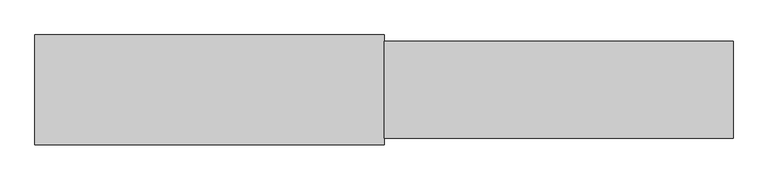
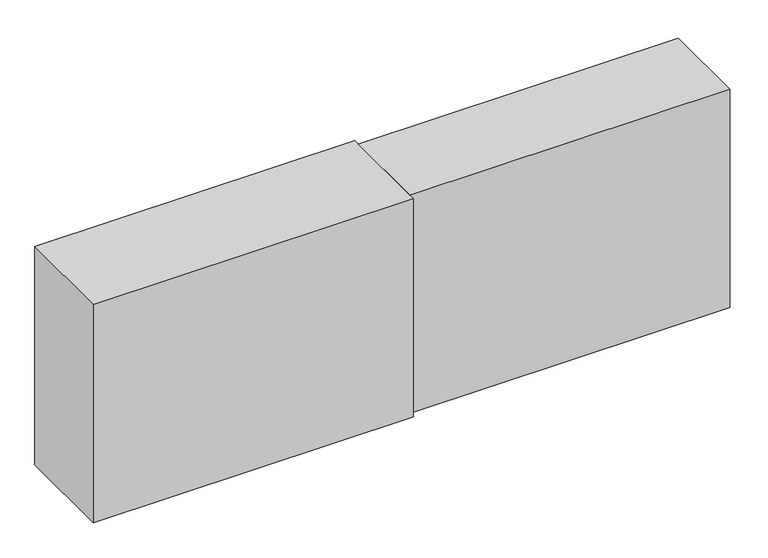
"""IFC4 building model written with IfcOpenShell, lengths in millimetres: proxy geometry, Тепловой пункт : Тепловой пункт."""

import ifcopenshell
import ifcopenshell.guid

model = None  # the IFC model being written
_history = None  # IfcOwnerHistory: only IFC2X3 demands one
_inside = {}  # id of a spatial element -> (the spatial element, [elements in it])
_under = {}  # id of a project, library or spatial element -> (it, [spatial elements below it])
_declared = {}  # id of a project -> (the project, [libraries it declares])
_typed = {}  # id of a type object -> (the type object, [elements of that type])
_made_of = {}  # id of a material, layer set ... -> (it, [elements and type objects made of it])


def new_model(schema):
    """Start an empty IFC model of exactly this schema.

    Asked for "IFC4X3", IfcOpenShell would pick the latest addendum, in which some entities
    have other attributes; the version numbers below select the first issue.
    IFC2X3 requires an IfcOwnerHistory on every rooted entity: one is made here for all.
    """
    global model, _history
    if schema == "IFC4X3":
        model = ifcopenshell.file(schema_version=(4, 3, 0, 0))
    else:
        model = ifcopenshell.file(schema=schema)
    _inside.clear()
    _under.clear()
    _declared.clear()
    _typed.clear()
    _made_of.clear()
    _history = None
    if model.schema == "IFC2X3":
        org = make("IfcOrganization", Name="unknown")
        user = make(
            "IfcPersonAndOrganization",
            ThePerson=make("IfcPerson", FamilyName="unknown"),
            TheOrganization=org,
        )
        app = make(
            "IfcApplication",
            ApplicationDeveloper=org,
            Version="unknown",
            ApplicationFullName="unknown",
            ApplicationIdentifier="unknown",
        )
        _history = make(
            "IfcOwnerHistory",
            OwningUser=user,
            OwningApplication=app,
            ChangeAction="ADDED",
            CreationDate=0,
        )
    return model


def make(cls, **values):
    """One entity of the class cls with the attributes given. An attribute that is None is left unset."""
    return model.create_entity(
        cls, **{name: value for name, value in values.items() if value is not None}
    )


def rooted(cls, **values):
    """An entity with a GlobalId (a new one), such as an element, a storey or a relation."""
    return make(cls, GlobalId=ifcopenshell.guid.new(), OwnerHistory=_history, **values)


def si_unit(unit_type, name, prefix=None):
    """IfcSIUnit, for example si_unit("LENGTHUNIT", "METRE", prefix="MILLI")."""
    return make("IfcSIUnit", UnitType=unit_type, Prefix=prefix, Name=name)


def assignment(units):
    """IfcUnitAssignment: the units of a project."""
    return None if units is None else make("IfcUnitAssignment", Units=units)


def point(xyz):
    """IfcCartesianPoint."""
    return None if xyz is None else make("IfcCartesianPoint", Coordinates=xyz)


def direction(xyz):
    """IfcDirection."""
    return None if xyz is None else make("IfcDirection", DirectionRatios=xyz)


def frame(location, z_axis=None, x_axis=None):
    """IfcAxis2Placement3D, a coordinate frame: its origin and axes. An axis left out is left unset."""
    return make(
        "IfcAxis2Placement3D",
        Location=point(location),
        Axis=direction(z_axis),
        RefDirection=direction(x_axis),
    )


def origin():
    """The frame at (0, 0, 0) with its axes left unset."""
    return frame((0.0, 0.0, 0.0))


def origin_with_axes():
    """The frame at (0, 0, 0) with the z axis (0, 0, 1) and the x axis (1, 0, 0) written out."""
    return frame((0.0, 0.0, 0.0), z_axis=(0.0, 0.0, 1.0), x_axis=(1.0, 0.0, 0.0))


def place(relative_to, where):
    """IfcLocalPlacement: puts the frame where relative to a parent placement (None: the world)."""
    return make(
        "IfcLocalPlacement", PlacementRelTo=relative_to, RelativePlacement=where
    )


def context(
    kind, dimensions, precision=None, world=None, true_north=None, identifier=None
):
    """IfcGeometricRepresentationContext, for example the 3D "Model" context."""
    return make(
        "IfcGeometricRepresentationContext",
        ContextIdentifier=identifier,
        ContextType=kind,
        CoordinateSpaceDimension=dimensions,
        Precision=precision,
        WorldCoordinateSystem=world,
        TrueNorth=true_north,
    )


def project(units=None, contexts=None):
    """IfcProject with its units and contexts."""
    return rooted(
        "IfcProject",
        Name="project",
        RepresentationContexts=contexts,
        UnitsInContext=assignment(units),
    )


def spatial(cls, under=None, at=None, **own):
    """A site, building, storey or space (cls), placed at a placement, below another one or the project."""
    s = rooted(cls, ObjectPlacement=at, **own)
    if under is not None:
        _under.setdefault(under.id(), (under, []))[1].append(s)
    return s


def polyline(points):
    """IfcPolyline through the points."""
    return make("IfcPolyline", Points=[point(p) for p in points])


def outline(outer, holes=None, kind="AREA"):
    """IfcArbitraryClosedProfileDef: a profile drawn as a closed curve; with holes, ...WithVoids."""
    if holes is None:
        return make("IfcArbitraryClosedProfileDef", ProfileType=kind, OuterCurve=outer)
    return make(
        "IfcArbitraryProfileDefWithVoids",
        ProfileType=kind,
        OuterCurve=outer,
        InnerCurves=holes,
    )


def extrude(swept, where, along, depth):
    """IfcExtrudedAreaSolid: the profile swept, set in the frame where, extruded along a direction by depth."""
    return make(
        "IfcExtrudedAreaSolid",
        SweptArea=swept,
        Position=where,
        ExtrudedDirection=direction(along),
        Depth=depth,
    )


def shape(context_of_items, identifier, shape_type, items):
    """IfcShapeRepresentation: the items that make up one representation, for example the "Body"."""
    return make(
        "IfcShapeRepresentation",
        ContextOfItems=context_of_items,
        RepresentationIdentifier=identifier,
        RepresentationType=shape_type,
        Items=items,
    )


def source(mapping_origin, context_of_items, identifier, shape_type, items):
    """IfcRepresentationMap: a shape defined once, which mapped items show again and again."""
    return make(
        "IfcRepresentationMap",
        MappingOrigin=mapping_origin,
        MappedRepresentation=shape(context_of_items, identifier, shape_type, items),
    )


def transform(
    local_origin,
    x_axis=None,
    y_axis=None,
    z_axis=None,
    scale=None,
    scale2=None,
    scale3=None,
    uniform=True,
):
    """IfcCartesianTransformationOperator3D, or its non-uniform kind. x_axis, y_axis, z_axis: its Axis1, 2, 3."""
    if uniform:
        return make(
            "IfcCartesianTransformationOperator3D",
            Axis1=direction(x_axis),
            Axis2=direction(y_axis),
            LocalOrigin=point(local_origin),
            Scale=scale,
            Axis3=direction(z_axis),
        )
    return make(
        "IfcCartesianTransformationOperator3DnonUniform",
        Axis1=direction(x_axis),
        Axis2=direction(y_axis),
        LocalOrigin=point(local_origin),
        Scale=scale,
        Axis3=direction(z_axis),
        Scale2=scale2,
        Scale3=scale3,
    )


def mapped(mapping_source, mapping_target):
    """IfcMappedItem: shows the shape of a source again, moved by a transform."""
    return make(
        "IfcMappedItem", MappingSource=mapping_source, MappingTarget=mapping_target
    )


def made_of(thing, what):
    """Note that an element or type object is made of a material, layer set ...; save() writes the relation."""
    if what is not None:
        _made_of.setdefault(what.id(), (what, []))[1].append(thing)
    return thing


def element(
    cls,
    number,
    at=None,
    inside=None,
    cuts=None,
    type_object=None,
    material=None,
    context=None,
    identifier="Body",
    shape_type=None,
    held_by="IfcProductDefinitionShape",
    body=None,
    shapes=None,
    **own,
):
    """One element of the class cls, such as IfcWall. Its Tag is "e" and its number.

    at: its placement. inside: the storey or other place that contains it. cuts: it is an
    opening in that element (IfcRelVoidsElement). A single representation is given by context,
    identifier, shape_type and body (its items); several are given by shapes. held_by: the class
    of the entity that holds the representations. save() writes the other relations.
    """
    e = rooted(cls, Tag="e%d" % number, ObjectPlacement=at, **own)
    if body is not None:
        shapes = [shape(context, identifier, shape_type, body)]
    if shapes is not None:
        e.Representation = make(held_by, Representations=shapes)
    if inside is not None:
        _inside.setdefault(inside.id(), (inside, []))[1].append(e)
    if cuts is not None:
        rooted(
            "IfcRelVoidsElement", RelatingBuildingElement=cuts, RelatedOpeningElement=e
        )
    if type_object is not None:
        _typed.setdefault(type_object.id(), (type_object, []))[1].append(e)
    return made_of(e, material)


def aggregate(whole, parts):
    """IfcRelAggregates: a whole, such as a stair, and the parts it consists of."""
    return rooted("IfcRelAggregates", RelatingObject=whole, RelatedObjects=parts)


def save(model, path):
    """Write the relations noted so far, then the file.

    IfcRelAggregates (storeys below a building ...), IfcRelContainedInSpatialStructure (elements
    in a storey), IfcRelDefinesByType, IfcRelAssociatesMaterial and IfcRelDeclares: one each for
    every whole, place, type object, material and project.
    """
    for whole, parts in _under.values():
        aggregate(whole, parts)
    for where, things in _inside.values():
        rooted(
            "IfcRelContainedInSpatialStructure",
            RelatedElements=things,
            RelatingStructure=where,
        )
    for kind, things in _typed.values():
        rooted("IfcRelDefinesByType", RelatedObjects=things, RelatingType=kind)
    for what, things in _made_of.values():
        rooted("IfcRelAssociatesMaterial", RelatedObjects=things, RelatingMaterial=what)
    for by, libraries in _declared.values():
        rooted("IfcRelDeclares", RelatingContext=by, RelatedDefinitions=libraries)
    model.write(path)


def generic_models_e1c33112(model_context):
    return source(origin(), model_context, "Body", "SweptSolid", [
        extrude(outline(polyline([(5400.0, 375.0), (5400.0, -375.0), (2700.0, -375.0), (2700.0, 375.0), (5400.0, 375.0)])), origin_with_axes(), (0.0, 0.0, 1.0), 1950.0),
        extrude(outline(polyline([(2700.0, 425.0), (2700.0, -425.0), (0.0, -425.0), (0.0, 425.0), (2700.0, 425.0)])), origin_with_axes(), (0.0, 0.0, 1.0), 1950.0),
    ])


if __name__ == "__main__":
    model = new_model("IFC4")
    model_context = context("Model", 3, world=origin())
    ifc_project = project(units=[si_unit("LENGTHUNIT", "METRE", prefix="MILLI")], contexts=[model_context])
    site = spatial("IfcSite", under=ifc_project)
    building = spatial("IfcBuilding", under=site)
    placement = place(None, origin())
    generic_models_shape = generic_models_e1c33112(model_context)
    element("IfcBuildingElementProxy", 1, Name="Тепловой пункт : Тепловой пункт", ObjectType="Тепловой пункт : Тепловой пункт", at=placement, inside=building, context=model_context, shape_type="MappedRepresentation", body=[
        mapped(generic_models_shape, transform((0.0, 0.0, 0.0), x_axis=(1.0, 0.0, 0.0), y_axis=(0.0, 1.0, 0.0), z_axis=(0.0, 0.0, 1.0))),
    ])
    save(model, "model.ifc")

# Revit data of these elements
# Type "Тепловой пункт : Тепловой пункт"
#   ADSK_Наименование = "Автоматизированный тепловой пункт"
#   Ширина узла ввода = 850 mm
#   Ширина модуль СО = 750 mm
#   Подключение к теплосети = 100 mm
#   Подключение к СО = 100 mm
#   Default Elevation = 0
